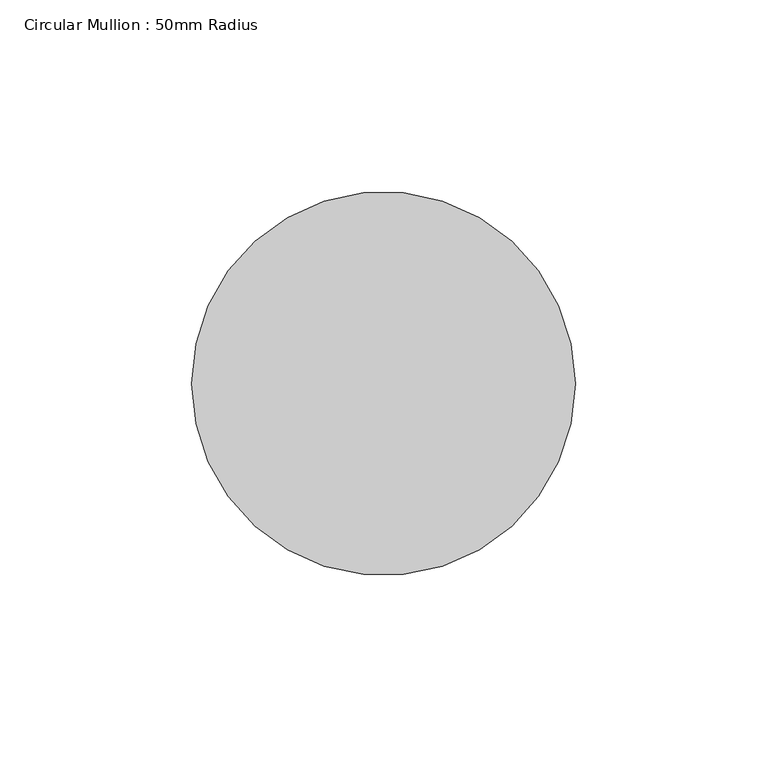
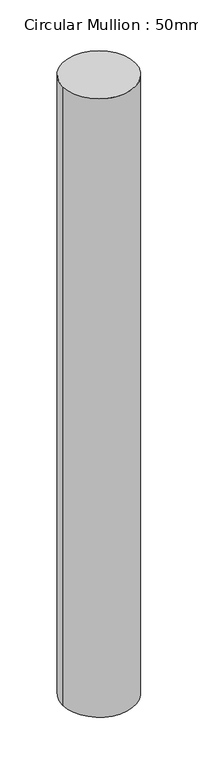
"""IFC4 building model written with IfcOpenShell, lengths in millimetres: member geometry, Circular Mullion : 50mm Radius."""

from ifc_helpers import new_model, si_unit, point, frame, origin, origin_2d, place, context, project, spatial, circle_curve, trimmed, segment, composite_curve, outline, extrude, source, transform, mapped, element, save


def circular_mullion_50mm_radius_7c53d19e(model_context):
    return source(origin(), model_context, "Body", "SweptSolid", [
        extrude(outline(composite_curve([segment(trimmed(circle_curve(origin_2d(), 50.0), [point((50.0, 0.0))], [point((-50.0, 0.0))], False, "CARTESIAN"), True, "CONTINUOUS"), segment(trimmed(circle_curve(origin_2d(), 50.0), [point((-50.0, 0.0))], [point((50.0, 0.0))], False, "CARTESIAN"), True, "CONTINUOUS")], self_intersect=False)), frame((0.0, 0.0, -900.8745106), z_axis=(0.0, 0.0, 1.0), x_axis=(1.0, 0.0, 0.0)), (0.0, 0.0, 1.0), 900.8745106),
    ])


if __name__ == "__main__":
    model = new_model("IFC4")
    model_context = context("Model", 3, world=origin())
    ifc_project = project(units=[si_unit("LENGTHUNIT", "METRE", prefix="MILLI")], contexts=[model_context])
    site = spatial("IfcSite", under=ifc_project)
    building = spatial("IfcBuilding", under=site)
    placement = place(None, origin())
    circular_mullion_50mm_radius_shape = circular_mullion_50mm_radius_7c53d19e(model_context)
    element("IfcMember", 1, ObjectType="Circular Mullion : 50mm Radius", at=placement, inside=building, context=model_context, shape_type="MappedRepresentation", body=[
        mapped(circular_mullion_50mm_radius_shape, transform((0.0, 0.0, 0.0), x_axis=(1.0, 0.0, 0.0), y_axis=(0.0, 1.0, 0.0), z_axis=(0.0, 0.0, 1.0))),
    ])
    save(model, "model.ifc")

# Revit data of these elements
# Type "Circular Mullion : 50mm Radius"
#   built-in parameter 1007350 = 0.164042 (stored number, unit not read)
# Element 1 (IfcMember, "Circular Mullion : 50mm Radius")
#   Materials on its faces: "Aluminium"
# Materials
#   "Aluminium": class "Metal", colour RGB 247 247 247, transparency 0, Description = "Aluminium 6061", Cost = 0
